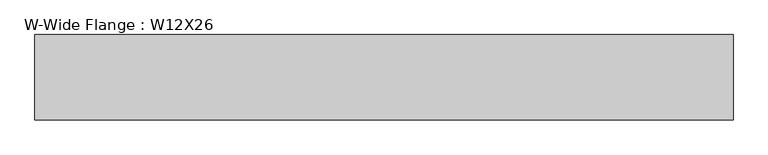
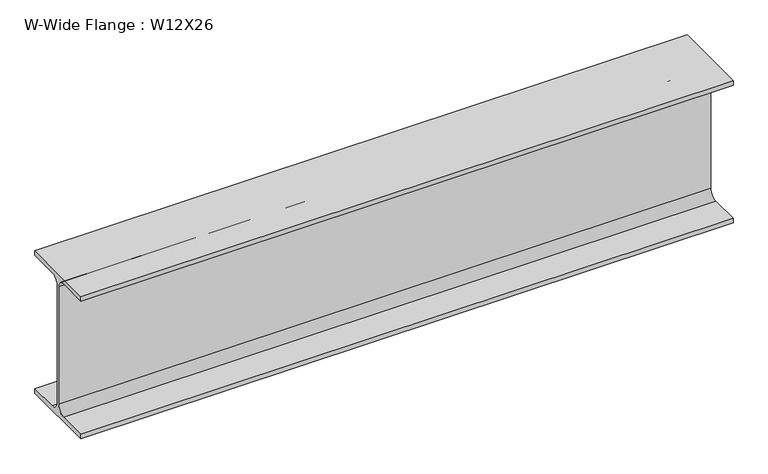
"""IFC4 building model written with IfcOpenShell, lengths in millimetres: beam geometry, W-Wide Flange : W12X26."""

from ifc_helpers import new_model, si_unit, point, frame, frame_2d, origin, place, context, project, spatial, polyline, circle_curve, trimmed, segment, composite_curve, outline, extrude, source, transform, mapped, element, save


def w_wide_flange_w12x26_c8fad4fd(model_context):
    return source(origin(), model_context, "Body", "SweptSolid", [
        extrude(outline(composite_curve([segment(polyline([(-82.4011719, -145.5539063), (-20.2902344, -145.5539063)]), True, "CONTINUOUS"), segment(trimmed(circle_curve(frame_2d((-20.2902344, -128.190625)), 17.3632812), [point((-20.2902344, -145.5539063))], [point((-2.9269531, -128.190625))], True, "CARTESIAN"), True, "CONTINUOUS"), segment(polyline([(-2.9269531, -128.190625), (-2.9269531, 128.190625)]), True, "CONTINUOUS"), segment(trimmed(circle_curve(frame_2d((-20.2902344, 128.190625)), 17.3632812), [point((-2.9269531, 128.190625))], [point((-20.2902344, 145.5539062))], True, "CARTESIAN"), True, "CONTINUOUS"), segment(polyline([(-20.2902344, 145.5539062), (-82.4011719, 145.5539062), (-82.4011719, 155.178125), (82.4011719, 155.178125), (82.4011719, 145.5539062), (20.2902344, 145.5539062)]), True, "CONTINUOUS"), segment(trimmed(circle_curve(frame_2d((20.2902344, 128.190625)), 17.3632812), [point((20.2902344, 145.5539062))], [point((2.9269531, 128.190625))], True, "CARTESIAN"), True, "CONTINUOUS"), segment(polyline([(2.9269531, 128.190625), (2.9269531, -128.190625)]), True, "CONTINUOUS"), segment(trimmed(circle_curve(frame_2d((20.2902344, -128.190625)), 17.3632812), [point((2.9269531, -128.190625))], [point((20.2902344, -145.5539063))], True, "CARTESIAN"), True, "CONTINUOUS"), segment(polyline([(20.2902344, -145.5539063), (82.4011719, -145.5539063), (82.4011719, -155.178125), (-82.4011719, -155.178125), (-82.4011719, -145.5539063)]), True, "CONTINUOUS")], self_intersect=False)), frame((-666.8988281, 0.0, 0.0), z_axis=(1.0, 0.0, 0.0), x_axis=(0.0, 1.0, 0.0)), (0.0, 0.0, 1.0), 1346.3488281),
    ])


if __name__ == "__main__":
    model = new_model("IFC4")
    model_context = context("Model", 3, world=origin())
    ifc_project = project(units=[si_unit("LENGTHUNIT", "METRE", prefix="MILLI")], contexts=[model_context])
    site = spatial("IfcSite", under=ifc_project)
    building = spatial("IfcBuilding", under=site)
    placement = place(None, origin())
    w_wide_flange_w12x26_shape = w_wide_flange_w12x26_c8fad4fd(model_context)
    element("IfcBeam", 1, ObjectType="W-Wide Flange : W12X26", at=placement, inside=building, context=model_context, shape_type="MappedRepresentation", body=[
        mapped(w_wide_flange_w12x26_shape, transform((0.0, 0.0, 0.0), x_axis=(1.0, 0.0, 0.0), y_axis=(0.0, 1.0, 0.0), z_axis=(0.0, 0.0, 1.0))),
    ])
    save(model, "model.ifc")

# Revit data of these elements
# Type "W-Wide Flange : W12X26"
#   Assembly Code = "B10"
#   W = 26
#   Start Extension Calculation [instance default] = 10' - 0"
#   Start Extension [instance default] = -0' - 0 1/2"
#   End Extension Calculation [instance default] = 10' - 0"
#   End Extension [instance default] = -0' - 0 1/2"
#   Length [instance default] = 5' - 0"
#   bf = 0' - 6 125/256"
#   d = 1' - 0 7/32"
#   k = 0' - 1 1/16"
#   k2 = 0' - 0 175/256"
#   tf = 0' - 0 97/256"
#   tw = 0' - 0 59/256"
#   A = 0.05 SF
#   Beam Material [instance default] = Metal - Steel - ASTM A992
# Element 1 (IfcBeam, "W-Wide Flange : W12X26")
#   Materials on its faces: "Metal - Steel - ASTM A992"
# Materials
#   "Metal - Steel - ASTM A992": class "Metal", colour RGB 128 0 0, transparency 0
